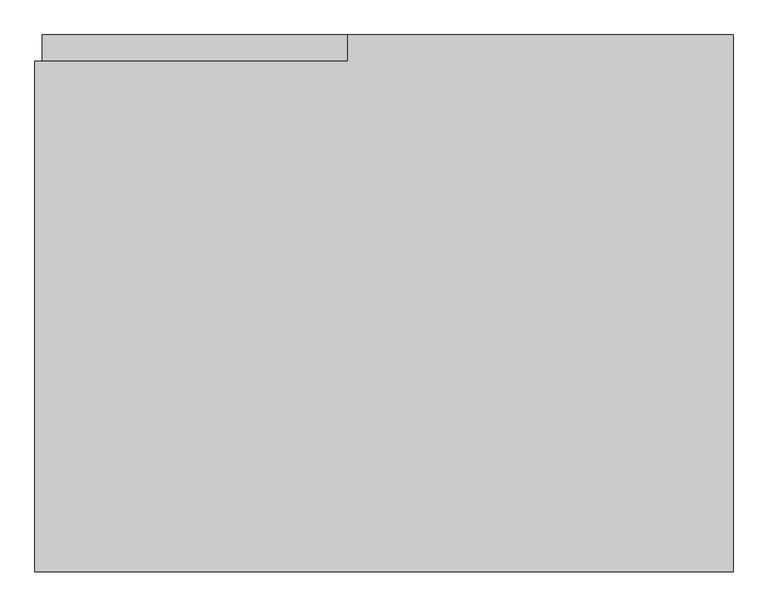
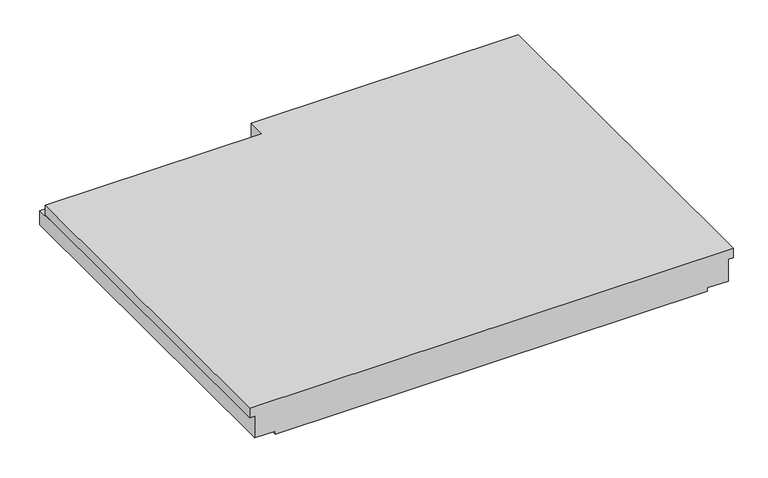
"""IFC4 building model written with IfcOpenShell, lengths in millimetres: proxy geometry, NLRS_24_GM_UN_rechthoekig bordes prefab zonder oplegnok-AV_gen_rsf : prefab bordes_gen__2250x2925."""

from ifc_helpers import new_model, si_unit, origin, place, context, project, spatial, faceted_brep, source, transform, mapped, element, save


def generic_models_1f2f9ad8(model_context):
    return source(origin(), model_context, "Body", "Brep", [
        faceted_brep([(1462.5, 2250.0, 0.0), (1462.5, 0.0, 0.0), (1462.5, 0.0, -60.0), (1462.5, 2250.0, -60.0), (-152.5, 2250.0, 0.0), (-152.5, 2250.0, -110.0), (-152.5, 2140.0, -110.0), (-152.5, 2140.0, 0.0), (-1462.5, 0.0, 0.0), (-1462.5, 2140.0, 0.0), (-1462.5, 2140.0, -60.0), (-1462.5, 0.0, -60.0), (-1432.5, 2250.0, -110.0), (1432.5, 2250.0, -60.0), (1432.5, 2250.0, -200.0), (1307.5, 2250.0, -200.0), (1307.5, 2250.0, -220.0), (-1307.5, 2250.0, -220.0), (-1307.5, 2250.0, -200.0), (-1432.5, 2250.0, -200.0), (-1432.5, 2140.0, -110.0), (-1432.5, 2140.0, -60.0), (-1432.5, 0.0, -60.0), (-1432.5, 0.0, -200.0), (-1307.5, 0.0, -200.0), (-1307.5, 0.0, -220.0), (1307.5, 0.0, -220.0), (1307.5, 0.0, -200.0), (1432.5, 0.0, -200.0), (1432.5, 0.0, -60.0)], [[[0, 1, 2, 3]], [[4, 5, 6, 7]], [[8, 9, 10, 11]], [[12, 5, 4, 0, 3, 13, 14, 15, 16, 17, 18, 19]], [[5, 12, 20, 6]], [[9, 7, 6, 20, 21, 10]], [[9, 8, 1, 0, 4, 7]], [[8, 11, 22, 23, 24, 25, 26, 27, 28, 29, 2, 1]], [[25, 17, 16, 26]], [[21, 22, 11, 10]], [[19, 23, 22, 21, 20, 12]], [[23, 19, 18, 24]], [[24, 18, 17, 25]], [[29, 13, 3, 2]], [[13, 29, 28, 14]], [[14, 28, 27, 15]], [[15, 27, 26, 16]]]),
    ])


if __name__ == "__main__":
    model = new_model("IFC4")
    model_context = context("Model", 3, world=origin())
    ifc_project = project(units=[si_unit("LENGTHUNIT", "METRE", prefix="MILLI")], contexts=[model_context])
    site = spatial("IfcSite", under=ifc_project)
    building = spatial("IfcBuilding", under=site)
    placement = place(None, origin())
    generic_models_shape = generic_models_1f2f9ad8(model_context)
    element("IfcBuildingElementProxy", 1, Name="NLRS_24_GM_UN_rechthoekig bordes prefab zonder oplegnok-AV_gen_rsf : prefab bordes_gen__2250x2925", ObjectType="NLRS_24_GM_UN_rechthoekig bordes prefab zonder oplegnok-AV_gen_rsf : prefab bordes_gen__2250x2925", at=placement, inside=building, context=model_context, shape_type="MappedRepresentation", body=[
        mapped(generic_models_shape, transform((0.0, 0.0, 0.0), x_axis=(1.0, 0.0, 0.0), y_axis=(0.0, 1.0, 0.0), z_axis=(0.0, 0.0, 1.0))),
    ])
    save(model, "model.ifc")

# Revit data of these elements
# Type "NLRS_24_GM_UN_rechthoekig bordes prefab zonder oplegnok-AV_gen_rsf : prefab bordes_gen__2250x2925"
#   Export Type to IFC As = "IfcStair"
#   Type IfcGUID = "2CEqVLPNH8KRN7ghwV3bOu"
#   Type Comments = " "
#   Model = " "
#   Manufacturer = " "
#   Description = "rechthoekig bordes prefab\r\n1930x4395"
#   Assembly Code = "24.15"
#   Width = 2925 mm
#   Thickness = 220 mm
#   Perimeter = 10350 mm
#   NLRS_C_lengte_02 = 1310 mm
#   NLRS_C_lengte_01 = 1310 mm
#   NLRS_C_hoogte_02 = 110 mm
#   NLRS_C_hoogte_01 = 110 mm
#   NLRS_C_diepte_04 = 2250 mm
#   NLRS_C_diepte_03 = 2250 mm
#   NLRS_C_diepte_02 = 110 mm
#   NLRS_C_diepte_01 = 110 mm
#   Length = 2250 mm
#   Default Elevation = 1219.2 mm
#   Area = 6.58125 m²
#   NLRS_C_materiaal = NLRS_f2_beton prefab_gen_rsf
#   Keynote = ""
# Element 1 (IfcBuildingElementProxy, "NLRS_24_GM_UN_rechthoekig bordes prefab zonder oplegnok-AV_gen_rsf : prefab bordes_gen__2250x2925")
#   Materials on its faces: "NLRS_f2_beton prefab_gen_rsf"
# Materials
#   "NLRS_f2_beton prefab_gen_rsf": class "F - Niet gebakken kunststeen", colour RGB 129 133 118, transparency 0, Keynote = "f2", Manufacturer = "Revit Standards Foundation", URL = "www.revitstandards.org", Description = "beton prefab", Cost = 0
